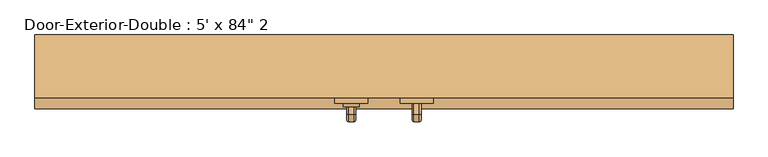
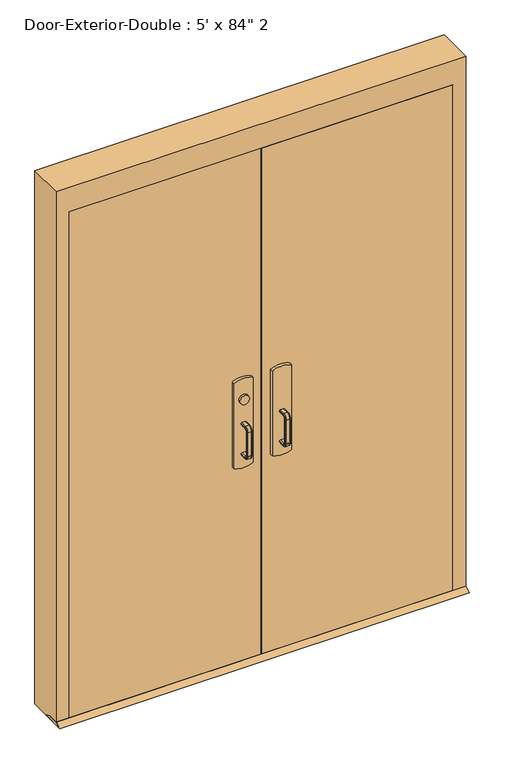
"""IFC4 building model written with IfcOpenShell, lengths in millimetres: door geometry."""

from ifc_helpers import new_model, si_unit, point, frame, frame_2d, origin, place, context, project, spatial, polyline, circle_curve, ellipse_curve, trimmed, segment, composite_curve, outline, extrude, faceted_brep, source, transform, mapped, element, save
from ifc_brep_helpers import plane_surface, cylinder_surface, revolved_surface, advanced_brep


def door_253b1ced(model_context):
    return source(origin(), model_context, "Body", "SolidModel", [
        extrude(outline(polyline([(-474.1333333, 12.7), (-76.2, 12.7), (-76.2, 6.35), (-474.1333333, 6.35), (-474.1333333, 12.7)])), frame((0.0, 0.0, 990.6), z_axis=(0.0, 0.0, 1.0), x_axis=(1.0, 0.0, 0.0)), (0.0, 0.0, 1.0), 50.8),
        advanced_brep(
        [(-12.7, 6.35, 1041.4), (-12.7, 6.35, 990.6), (-76.2, 6.35, 990.6), (-673.1, 6.35, 990.6), (-673.1, 6.35, 1041.4), (-76.2, 6.35, 1041.4), (-673.1, -25.4, 1041.4), (-673.1, -25.4, 990.6), (-76.2, -25.4, 990.6), (-76.2, -25.4, 927.1), (-57.15, -25.4, 908.05), (-31.75, -25.4, 908.05), (-12.7, -25.4, 927.1), (-12.7, -25.4, 1104.9), (-31.75, -25.4, 1123.95), (-57.15, -25.4, 1123.95), (-76.2, -25.4, 1104.9), (-76.2, -25.4, 1041.4), (-76.2, 3.1747533, 1041.4), (-12.7, 3.1747533, 1041.4), (-12.7, -1.8354269, 1104.9), (-12.7, -1.8354269, 927.1), (-12.7, 3.1747533, 990.6), (-76.2, 3.1747533, 990.6), (-76.2, -1.8354269, 1104.9), (-76.2, -1.8354269, 927.1), (-31.75, -3.338481, 1123.95), (-57.15, -3.338481, 1123.95), (-57.15, -3.338481, 908.05), (-31.75, -3.338481, 908.05)],
        [
            (0, 1),
            (1, 2),
            (2, 3),
            (3, 4),
            (4, 5),
            (5, 0),
            (6, 7),
            (7, 8),
            (8, 9),
            (9, 10, circle_curve(frame((-57.15, -25.4, 927.1), z_axis=(0.0, -1.0, 0.0), x_axis=(-1.0, 0.0, 0.0)), 19.05)),
            (10, 11),
            (11, 12, circle_curve(frame((-31.75, -25.4, 927.1), z_axis=(0.0, -1.0, 0.0), x_axis=(-1.0, 0.0, 0.0)), 19.05)),
            (12, 13),
            (13, 14, circle_curve(frame((-31.75, -25.4, 1104.9), z_axis=(0.0, -1.0, 0.0), x_axis=(-1.0, 0.0, 0.0)), 19.05)),
            (14, 15),
            (15, 16, circle_curve(frame((-57.15, -25.4, 1104.9), z_axis=(0.0, -1.0, 0.0), x_axis=(-1.0, 0.0, 0.0)), 19.05)),
            (16, 17),
            (17, 6),
            (4, 6),
            (17, 18),
            (18, 19),
            (19, 0),
            (19, 20),
            (20, 13),
            (12, 21),
            (21, 22),
            (22, 1),
            (7, 3),
            (22, 23),
            (23, 8),
            (16, 24),
            (24, 18),
            (23, 25),
            (25, 9),
            (14, 26),
            (26, 27),
            (27, 15),
            (10, 28),
            (28, 29),
            (29, 11),
            (25, 28, ellipse_curve(frame((-57.15, -1.8354269, 927.1), z_axis=(0.0, -0.9969018152893365, 0.07865602756830282), x_axis=(0.0, 0.07865602756830208, 0.9969018152893365)), 19.1092038, 19.05)),
            (27, 24, ellipse_curve(frame((-57.15, -1.8354269, 1104.9), z_axis=(0.0, -0.9969018152893376, -0.07865602756828934), x_axis=(0.0, 0.078656027568288, -0.9969018152893377)), 19.1092038, 19.05)),
            (20, 26, ellipse_curve(frame((-31.75, -1.8354269, 1104.9), z_axis=(0.0, -0.9969018152893376, -0.07865602756828934), x_axis=(0.0, 0.078656027568288, -0.9969018152893377)), 19.1092038, 19.05)),
            (29, 21, ellipse_curve(frame((-31.75, -1.8354269, 927.1), z_axis=(0.0, -0.9969018152893365, 0.07865602756830282), x_axis=(0.0, 0.07865602756830208, 0.9969018152893365)), 19.1092038, 19.05)),
        ],
        [
            plane_surface(frame((-12.7, 6.35, 1041.4), z_axis=(0.0, 1.0, 0.0), x_axis=(1.0, 0.0, 0.0))),
            plane_surface(frame((-12.7, -25.4, 1041.4), z_axis=(0.0, -1.0, 0.0), x_axis=(-1.0, 0.0, 0.0))),
            plane_surface(frame((-673.1, 6.35, 1041.4), z_axis=(0.0, 0.0, 1.0), x_axis=(0.0, -1.0, 0.0))),
            plane_surface(frame((-12.7, 6.35, 1041.4), z_axis=(1.0, 0.0, 0.0), x_axis=(0.0, -1.0, 0.0))),
            plane_surface(frame((-12.7, 6.35, 990.6), z_axis=(0.0, 0.0, -1.0), x_axis=(0.0, -1.0, 0.0))),
            plane_surface(frame((-673.1, 6.35, 990.6), z_axis=(-1.0, 0.0, 0.0), x_axis=(0.0, -1.0, 0.0))),
            plane_surface(frame((-76.2, 3.1747533, 927.1), z_axis=(-1.0, 0.0, 0.0), x_axis=(0.0, -1.0, 0.0))),
            plane_surface(frame((-57.15, 3.1747533, 1123.95), z_axis=(0.0, 0.0, 1.0), x_axis=(0.0, -1.0, 0.0))),
            plane_surface(frame((-31.75, 3.1747533, 908.05), z_axis=(0.0, 0.0, -1.0), x_axis=(0.0, -1.0, 0.0))),
            cylinder_surface(frame((-57.15, -25.4, 927.1), z_axis=(0.0, 1.0, 0.0), x_axis=(-1.0, 0.0, 0.0)), 19.05),
            cylinder_surface(frame((-57.15, -25.4, 1104.9), z_axis=(0.0, 1.0, 0.0), x_axis=(-1.0, 0.0, 0.0)), 19.05),
            cylinder_surface(frame((-31.75, -25.4, 1104.9), z_axis=(0.0, 1.0, 0.0), x_axis=(-1.0, 0.0, 0.0)), 19.05),
            cylinder_surface(frame((-31.75, -25.4, 927.1), z_axis=(0.0, 1.0, 0.0), x_axis=(-1.0, 0.0, 0.0)), 19.05),
            plane_surface(frame((-76.2, 3.1747533, 1041.4), z_axis=(0.0, 0.9969018152893376, 0.07865602756828934), x_axis=(1.0, 0.0, 0.0))),
            plane_surface(frame((-76.2, -3.338481, 908.05), z_axis=(0.0, 0.9969018152893365, -0.07865602756830282), x_axis=(1.0, 0.0, 0.0))),
        ],
        [
            (0, [[1, 2, 3, 4, 5, 6]]),
            (1, [[7, 8, 9, 10, 11, 12, 13, 14, 15, 16, 17, 18]]),
            (2, [[19, -18, 20, 21, 22, -6, -5]]),
            (3, [[-1, -22, 23, 24, -13, 25, 26, 27]]),
            (4, [[28, -3, -2, -27, 29, 30, -8]]),
            (5, [[-4, -28, -7, -19]]),
            (6, [[-17, 31, 32, -20]]),
            (6, [[-9, -30, 33, 34]]),
            (7, [[-15, 35, 36, 37]]),
            (8, [[-11, 38, 39, 40]]),
            (9, [[-10, -34, 41, -38]]),
            (10, [[-16, -37, 42, -31]]),
            (11, [[-14, -24, 43, -35]]),
            (12, [[-12, -40, 44, -25]]),
            (13, [[-21, -32, -42, -36, -43, -23]]),
            (14, [[-26, -44, -39, -41, -33, -29]]),
        ],
    ),
        extrude(outline(polyline([(-69.85, 12.7), (-25.4, 12.7), (0.0, 0.0), (-95.25, 0.0), (-69.85, 12.7)])), frame((-812.8, 0.0, 0.0), z_axis=(1.0, 0.0, 0.0), x_axis=(0.0, 1.0, 0.0)), (0.0, 0.0, 1.0), 1625.6),
        extrude(outline(polyline([(474.1333333, 12.7), (474.1333333, 6.35), (76.2, 6.35), (76.2, 12.7), (474.1333333, 12.7)])), frame((0.0, 0.0, 990.6), z_axis=(0.0, 0.0, 1.0), x_axis=(1.0, 0.0, 0.0)), (0.0, 0.0, 1.0), 50.8),
        advanced_brep(
        [(12.7, 6.35, 1041.4), (76.2, 6.35, 1041.4), (673.1, 6.35, 1041.4), (673.1, 6.35, 990.6), (76.2, 6.35, 990.6), (12.7, 6.35, 990.6), (673.1, -25.4, 1041.4), (76.2, -25.4, 1041.4), (76.2, -25.4, 1104.9), (57.15, -25.4, 1123.95), (31.75, -25.4, 1123.95), (12.7, -25.4, 1104.9), (12.7, -25.4, 927.1), (31.75, -25.4, 908.05), (57.15, -25.4, 908.05), (76.2, -25.4, 927.1), (76.2, -25.4, 990.6), (673.1, -25.4, 990.6), (12.7, 3.1747533, 1041.4), (76.2, 3.1747533, 1041.4), (12.7, 3.1747533, 990.6), (12.7, -1.8354269, 927.1), (12.7, -1.8354269, 1104.9), (76.2, 3.1747533, 990.6), (76.2, -1.8354269, 1104.9), (76.2, -1.8354269, 927.1), (57.15, -3.338481, 1123.95), (31.75, -3.338481, 1123.95), (31.75, -3.338481, 908.05), (57.15, -3.338481, 908.05)],
        [
            (0, 1),
            (1, 2),
            (2, 3),
            (3, 4),
            (4, 5),
            (5, 0),
            (6, 7),
            (7, 8),
            (8, 9, circle_curve(frame((57.15, -25.4, 1104.9), z_axis=(0.0, -1.0, 0.0), x_axis=(1.0, 0.0, 0.0)), 19.05)),
            (9, 10),
            (10, 11, circle_curve(frame((31.75, -25.4, 1104.9), z_axis=(0.0, -1.0, 0.0), x_axis=(1.0, 0.0, 0.0)), 19.05)),
            (11, 12),
            (12, 13, circle_curve(frame((31.75, -25.4, 927.1), z_axis=(0.0, -1.0, 0.0), x_axis=(1.0, 0.0, 0.0)), 19.05)),
            (13, 14),
            (14, 15, circle_curve(frame((57.15, -25.4, 927.1), z_axis=(0.0, -1.0, 0.0), x_axis=(1.0, 0.0, 0.0)), 19.05)),
            (15, 16),
            (16, 17),
            (17, 6),
            (0, 18),
            (18, 19),
            (19, 7),
            (6, 2),
            (5, 20),
            (20, 21),
            (21, 12),
            (11, 22),
            (22, 18),
            (16, 23),
            (23, 20),
            (3, 17),
            (19, 24),
            (24, 8),
            (15, 25),
            (25, 23),
            (9, 26),
            (26, 27),
            (27, 10),
            (13, 28),
            (28, 29),
            (29, 14),
            (29, 25, ellipse_curve(frame((57.15, -1.8354269, 927.1), z_axis=(0.0, -0.9969018152893365, 0.07865602756830282), x_axis=(0.0, 0.07865602756830208, 0.9969018152893365)), 19.1092038, 19.05)),
            (24, 26, ellipse_curve(frame((57.15, -1.8354269, 1104.9), z_axis=(0.0, -0.9969018152893376, -0.07865602756828934), x_axis=(0.0, 0.078656027568288, -0.9969018152893377)), 19.1092038, 19.05)),
            (27, 22, ellipse_curve(frame((31.75, -1.8354269, 1104.9), z_axis=(0.0, -0.9969018152893376, -0.07865602756828934), x_axis=(0.0, 0.078656027568288, -0.9969018152893377)), 19.1092038, 19.05)),
            (21, 28, ellipse_curve(frame((31.75, -1.8354269, 927.1), z_axis=(0.0, -0.9969018152893365, 0.07865602756830282), x_axis=(0.0, 0.07865602756830208, 0.9969018152893365)), 19.1092038, 19.05)),
        ],
        [
            plane_surface(frame((12.7, 6.35, 1041.4), z_axis=(0.0, 1.0, 0.0), x_axis=(-1.0, 0.0, 0.0))),
            plane_surface(frame((12.7, -25.4, 1041.4), z_axis=(0.0, -1.0, 0.0), x_axis=(1.0, 0.0, 0.0))),
            plane_surface(frame((673.1, 6.35, 1041.4), z_axis=(0.0, 0.0, 1.0), x_axis=(0.0, -1.0, 0.0))),
            plane_surface(frame((12.7, 6.35, 1041.4), z_axis=(-1.0, 0.0, 0.0), x_axis=(0.0, -1.0, 0.0))),
            plane_surface(frame((12.7, 6.35, 990.6), z_axis=(0.0, 0.0, -1.0), x_axis=(0.0, -1.0, 0.0))),
            plane_surface(frame((673.1, 6.35, 990.6), z_axis=(1.0, 0.0, 0.0), x_axis=(0.0, -1.0, 0.0))),
            plane_surface(frame((76.2, 3.1747533, 927.1), z_axis=(1.0, 0.0, 0.0), x_axis=(0.0, -1.0, 0.0))),
            plane_surface(frame((57.15, 3.1747533, 1123.95), z_axis=(0.0, 0.0, 1.0), x_axis=(0.0, -1.0, 0.0))),
            plane_surface(frame((31.75, 3.1747533, 908.05), z_axis=(0.0, 0.0, -1.0), x_axis=(0.0, -1.0, 0.0))),
            cylinder_surface(frame((57.15, -25.4, 927.1), z_axis=(0.0, 1.0, 0.0), x_axis=(1.0, 0.0, 0.0)), 19.05),
            cylinder_surface(frame((57.15, -25.4, 1104.9), z_axis=(0.0, 1.0, 0.0), x_axis=(1.0, 0.0, 0.0)), 19.05),
            cylinder_surface(frame((31.75, -25.4, 1104.9), z_axis=(0.0, 1.0, 0.0), x_axis=(1.0, 0.0, 0.0)), 19.05),
            cylinder_surface(frame((31.75, -25.4, 927.1), z_axis=(0.0, 1.0, 0.0), x_axis=(1.0, 0.0, 0.0)), 19.05),
            plane_surface(frame((76.2, 3.1747533, 1041.4), z_axis=(0.0, 0.9969018152893376, 0.07865602756828934), x_axis=(-1.0, 0.0, 0.0))),
            plane_surface(frame((76.2, -3.338481, 908.05), z_axis=(0.0, 0.9969018152893365, -0.07865602756830282), x_axis=(-1.0, 0.0, 0.0))),
        ],
        [
            (0, [[1, 2, 3, 4, 5, 6]]),
            (1, [[7, 8, 9, 10, 11, 12, 13, 14, 15, 16, 17, 18]]),
            (2, [[-2, -1, 19, 20, 21, -7, 22]]),
            (3, [[23, 24, 25, -12, 26, 27, -19, -6]]),
            (4, [[-17, 28, 29, -23, -5, -4, 30]]),
            (5, [[-22, -18, -30, -3]]),
            (6, [[-21, 31, 32, -8]]),
            (6, [[33, 34, -28, -16]]),
            (7, [[35, 36, 37, -10]]),
            (8, [[38, 39, 40, -14]]),
            (9, [[-40, 41, -33, -15]]),
            (10, [[-32, 42, -35, -9]]),
            (11, [[-37, 43, -26, -11]]),
            (12, [[-25, 44, -38, -13]]),
            (13, [[-27, -43, -36, -42, -31, -20]]),
            (14, [[-29, -34, -41, -39, -44, -24]]),
        ],
    ),
        advanced_brep(
        [(66.2, -82.55, 1017.190625), (69.771875, -82.55, 1020.7625), (82.628125, -82.55, 1020.7625), (86.2, -82.55, 1017.190625), (86.2, -82.55, 1014.8090406), (82.6284594, -82.55, 1011.2375), (69.771875, -82.55, 1011.2375), (66.2, -82.55, 1014.809375), (66.2, -82.55, 887.809375), (66.2, -82.55, 890.190625), (69.771875, -82.55, 893.7625), (82.6284594, -82.55, 893.7625), (86.2, -82.55, 890.1909594), (86.2, -82.55, 887.809375), (82.628125, -82.55, 884.2375), (69.771875, -82.55, 884.2375), (66.2, -107.95, 1014.809375), (66.2, -119.459375, 1003.3), (66.2, -119.459375, 901.7), (66.2, -107.95, 890.190625), (66.2, -107.95, 887.809375), (66.2, -121.840625, 901.7), (66.2, -121.840625, 1003.3), (66.2, -107.95, 1017.190625), (69.771875, -107.95, 1011.2375), (82.6284594, -107.95, 1011.2375), (86.2, -107.95, 1014.8090406), (86.2, -107.95, 1017.190625), (86.2, -121.840625, 1003.3), (86.2, -121.840625, 901.7), (86.2, -107.95, 887.809375), (86.2, -107.95, 890.1909594), (86.2, -119.4590406, 901.7), (86.2, -119.4590406, 1003.3), (82.628125, -107.95, 1020.7625), (69.771875, -107.95, 1020.7625), (69.771875, -115.8875, 1003.3), (82.6284594, -115.8875, 1003.3), (82.628125, -125.4125, 1003.3), (69.771875, -125.4125, 1003.3), (69.771875, -115.8875, 901.7), (82.6284594, -115.8875, 901.7), (82.628125, -125.4125, 901.7), (69.771875, -125.4125, 901.7), (69.771875, -107.95, 893.7625), (82.6284594, -107.95, 893.7625), (82.628125, -107.95, 884.2375), (69.771875, -107.95, 884.2375)],
        [
            (0, 1, circle_curve(frame((69.771875, -82.55, 1017.190625), z_axis=(0.0, 1.0, 0.0), x_axis=(0.0, 0.0, 1.0)), 3.571875)),
            (1, 2),
            (2, 3, circle_curve(frame((82.628125, -82.55, 1017.190625), z_axis=(0.0, 1.0, 0.0), x_axis=(0.0, 0.0, 1.0)), 3.571875)),
            (3, 4),
            (4, 5, circle_curve(frame((82.6284594, -82.55, 1014.8090406), z_axis=(0.0, 1.0, 0.0), x_axis=(0.0, 0.0, 1.0)), 3.5715406)),
            (5, 6),
            (6, 7, circle_curve(frame((69.771875, -82.55, 1014.809375), z_axis=(0.0, 1.0, 0.0), x_axis=(0.0, 0.0, 1.0)), 3.571875)),
            (7, 0),
            (8, 9),
            (9, 10, circle_curve(frame((69.771875, -82.55, 890.190625), z_axis=(0.0, 1.0, 0.0), x_axis=(0.0, 0.0, -1.0)), 3.571875)),
            (10, 11),
            (11, 12, circle_curve(frame((82.6284594, -82.55, 890.1909594), z_axis=(0.0, 1.0, 0.0), x_axis=(0.0, 0.0, -1.0)), 3.5715406)),
            (12, 13),
            (13, 14, circle_curve(frame((82.628125, -82.55, 887.809375), z_axis=(0.0, 1.0, 0.0), x_axis=(0.0, 0.0, -1.0)), 3.571875)),
            (14, 15),
            (15, 8, circle_curve(frame((69.771875, -82.55, 887.809375), z_axis=(0.0, 1.0, 0.0), x_axis=(0.0, 0.0, -1.0)), 3.571875)),
            (7, 16),
            (16, 17, circle_curve(frame((66.2, -107.95, 1003.3), z_axis=(1.0, 0.0, 0.0), x_axis=(0.0, 0.0, 1.0)), 11.509375)),
            (17, 18),
            (18, 19, circle_curve(frame((66.2, -107.95, 901.7), z_axis=(1.0, 0.0, 0.0), x_axis=(0.0, -1.0, 0.0)), 11.509375)),
            (19, 9),
            (8, 20),
            (20, 21, circle_curve(frame((66.2, -107.95, 901.7), z_axis=(-1.0, 0.0, 0.0), x_axis=(0.0, -1.0, 0.0)), 13.890625)),
            (21, 22),
            (22, 23, circle_curve(frame((66.2, -107.95, 1003.3), z_axis=(-1.0, 0.0, 0.0), x_axis=(0.0, 0.0, 1.0)), 13.890625)),
            (23, 0),
            (6, 24),
            (24, 16, circle_curve(frame((69.771875, -107.95, 1014.809375), z_axis=(0.0, 1.0, 0.0), x_axis=(0.0, 0.0, 1.0)), 3.571875)),
            (5, 25),
            (25, 24),
            (4, 26),
            (26, 25, circle_curve(frame((82.6284594, -107.95, 1014.8090406), z_axis=(0.0, 1.0, 0.0), x_axis=(0.0, 0.0, 1.0)), 3.5715406)),
            (3, 27),
            (27, 28, circle_curve(frame((86.2, -107.95, 1003.3), z_axis=(1.0, 0.0, 0.0), x_axis=(0.0, 0.0, 1.0)), 13.890625)),
            (28, 29),
            (29, 30, circle_curve(frame((86.2, -107.95, 901.7), z_axis=(1.0, 0.0, 0.0), x_axis=(0.0, -1.0, 0.0)), 13.890625)),
            (30, 13),
            (12, 31),
            (31, 32, circle_curve(frame((86.2, -107.95, 901.7), z_axis=(-1.0, 0.0, 0.0), x_axis=(0.0, -1.0, 0.0)), 11.5090406)),
            (32, 33),
            (33, 26, circle_curve(frame((86.2, -107.95, 1003.3), z_axis=(-1.0, 0.0, 0.0), x_axis=(0.0, 0.0, 1.0)), 11.5090406)),
            (2, 34),
            (34, 27, circle_curve(frame((82.628125, -107.95, 1017.190625), z_axis=(0.0, 1.0, 0.0), x_axis=(0.0, 0.0, 1.0)), 3.571875)),
            (1, 35),
            (35, 34),
            (23, 35, circle_curve(frame((69.771875, -107.95, 1017.190625), z_axis=(0.0, 1.0, 0.0), x_axis=(0.0, 0.0, 1.0)), 3.571875)),
            (36, 17, circle_curve(frame((69.771875, -119.459375, 1003.3), z_axis=(0.0, 0.0, 1.0), x_axis=(0.0, -1.0, 0.0)), 3.571875)),
            (24, 36, circle_curve(frame((69.771875, -107.95, 1003.3), z_axis=(1.0, 0.0, 0.0), x_axis=(0.0, 0.0, 1.0)), 7.9375)),
            (37, 36),
            (25, 37, circle_curve(frame((82.6284594, -107.95, 1003.3), z_axis=(1.0, 0.0, 0.0), x_axis=(0.0, 0.0, 1.0)), 7.9375)),
            (33, 37, circle_curve(frame((82.6284594, -119.4590406, 1003.3), z_axis=(0.0, 0.0, 1.0), x_axis=(0.0, -1.0, 0.0)), 3.5715406)),
            (38, 28, circle_curve(frame((82.628125, -121.840625, 1003.3), z_axis=(0.0, 0.0, 1.0), x_axis=(0.0, -1.0, 0.0)), 3.571875)),
            (34, 38, circle_curve(frame((82.628125, -107.95, 1003.3), z_axis=(1.0, 0.0, 0.0), x_axis=(0.0, 0.0, 1.0)), 17.4625)),
            (39, 38),
            (35, 39, circle_curve(frame((69.771875, -107.95, 1003.3), z_axis=(1.0, 0.0, 0.0), x_axis=(0.0, 0.0, 1.0)), 17.4625)),
            (22, 39, circle_curve(frame((69.771875, -121.840625, 1003.3), z_axis=(0.0, 0.0, 1.0), x_axis=(0.0, -1.0, 0.0)), 3.571875)),
            (36, 40),
            (40, 18, circle_curve(frame((69.771875, -119.459375, 901.7), z_axis=(0.0, 0.0, 1.0), x_axis=(0.0, -1.0, 0.0)), 3.571875)),
            (37, 41),
            (41, 40),
            (32, 41, circle_curve(frame((82.6284594, -119.4590406, 901.7), z_axis=(0.0, 0.0, 1.0), x_axis=(0.0, -1.0, 0.0)), 3.5715406)),
            (38, 42),
            (42, 29, circle_curve(frame((82.628125, -121.840625, 901.7), z_axis=(0.0, 0.0, 1.0), x_axis=(0.0, -1.0, 0.0)), 3.571875)),
            (39, 43),
            (43, 42),
            (21, 43, circle_curve(frame((69.771875, -121.840625, 901.7), z_axis=(0.0, 0.0, 1.0), x_axis=(0.0, -1.0, 0.0)), 3.571875)),
            (44, 19, circle_curve(frame((69.771875, -107.95, 890.190625), z_axis=(0.0, -1.0, 0.0), x_axis=(0.0, 0.0, -1.0)), 3.571875)),
            (40, 44, circle_curve(frame((69.771875, -107.95, 901.7), z_axis=(1.0, 0.0, 0.0), x_axis=(0.0, -1.0, 0.0)), 7.9375)),
            (45, 44),
            (41, 45, circle_curve(frame((82.6284594, -107.95, 901.7), z_axis=(1.0, 0.0, 0.0), x_axis=(0.0, -1.0, 0.0)), 7.9375)),
            (31, 45, circle_curve(frame((82.6284594, -107.95, 890.1909594), z_axis=(0.0, -1.0, 0.0), x_axis=(0.0, 0.0, -1.0)), 3.5715406)),
            (46, 30, circle_curve(frame((82.628125, -107.95, 887.809375), z_axis=(0.0, -1.0, 0.0), x_axis=(0.0, 0.0, -1.0)), 3.571875)),
            (42, 46, circle_curve(frame((82.628125, -107.95, 901.7), z_axis=(1.0, 0.0, 0.0), x_axis=(0.0, -1.0, 0.0)), 17.4625)),
            (47, 46),
            (43, 47, circle_curve(frame((69.771875, -107.95, 901.7), z_axis=(1.0, 0.0, 0.0), x_axis=(0.0, -1.0, 0.0)), 17.4625)),
            (20, 47, circle_curve(frame((69.771875, -107.95, 887.809375), z_axis=(0.0, -1.0, 0.0), x_axis=(0.0, 0.0, -1.0)), 3.571875)),
            (44, 10),
            (45, 11),
            (46, 14),
            (47, 15),
        ],
        [
            plane_surface(frame((76.2, -82.55, 1016.0), z_axis=(0.0, 1.0, 0.0), x_axis=(1.0, 0.0, 0.0))),
            plane_surface(frame((76.2, -82.55, 889.0), z_axis=(0.0, 1.0, 0.0), x_axis=(1.0, 0.0, 0.0))),
            plane_surface(frame((66.2, -82.55, 1017.190625), z_axis=(-1.0, 0.0, 0.0), x_axis=(0.0, -1.0, 0.0))),
            cylinder_surface(frame((69.771875, -82.55, 1014.809375), z_axis=(0.0, 1.0, 0.0), x_axis=(0.0, 0.0, 1.0)), 3.571875),
            plane_surface(frame((69.771875, -82.55, 1011.2375), z_axis=(0.0, 0.0, -1.0), x_axis=(0.0, -1.0, 0.0))),
            cylinder_surface(frame((82.6284594, -82.55, 1014.8090406), z_axis=(0.0, 1.0, 0.0), x_axis=(0.0, 0.0, 1.0)), 3.5715406),
            plane_surface(frame((86.2, -82.55, 1014.8090406), z_axis=(1.0, 0.0, 0.0), x_axis=(0.0, -1.0, 0.0))),
            cylinder_surface(frame((82.628125, -82.55, 1017.190625), z_axis=(0.0, 1.0, 0.0), x_axis=(0.0, 0.0, 1.0)), 3.571875),
            plane_surface(frame((82.628125, -82.55, 1020.7625), z_axis=(0.0, 0.0, 1.0), x_axis=(0.0, -1.0, 0.0))),
            cylinder_surface(frame((69.771875, -82.55, 1017.190625), z_axis=(0.0, 1.0, 0.0), x_axis=(0.0, 0.0, 1.0)), 3.571875),
            revolved_surface(trimmed(ellipse_curve(frame((69.771875, -107.95, 1014.809375), z_axis=(0.0, -1.0, 0.0), x_axis=(0.0, 0.0, 1.0)), 3.571875, 3.571875), [point((66.2, -107.95, 1014.809375))], [point((69.771875, -107.95, 1011.2375))], True, "CARTESIAN"), (76.2, -107.95, 1003.3), (-1.0, 0.0, 0.0)),
            revolved_surface(polyline([(69.771875, -107.95, 1011.2375), (82.6284594, -107.95, 1011.2375)]), (76.2, -107.95, 1003.3), (-1.0, 0.0, 0.0)),
            revolved_surface(trimmed(ellipse_curve(frame((82.6284594, -107.95, 1014.8090406), z_axis=(0.0, -1.0, 0.0), x_axis=(0.0, 0.0, 1.0)), 3.5715406, 3.5715406), [point((82.6284594, -107.95, 1011.2375))], [point((86.2, -107.95, 1014.8090406))], True, "CARTESIAN"), (76.2, -107.95, 1003.3), (-1.0, 0.0, 0.0)),
            revolved_surface(trimmed(ellipse_curve(frame((82.628125, -107.95, 1017.190625), z_axis=(0.0, -1.0, 0.0), x_axis=(0.0, 0.0, 1.0)), 3.571875, 3.571875), [point((86.2, -107.95, 1017.190625))], [point((82.628125, -107.95, 1020.7625))], True, "CARTESIAN"), (76.2, -107.95, 1003.3), (-1.0, 0.0, 0.0)),
            cylinder_surface(frame((76.2, -107.95, 1003.3), z_axis=(-1.0, 0.0, 0.0), x_axis=(0.0, 0.0, 1.0)), 17.4625),
            revolved_surface(trimmed(ellipse_curve(frame((69.771875, -107.95, 1017.190625), z_axis=(0.0, -1.0, 0.0), x_axis=(0.0, 0.0, 1.0)), 3.571875, 3.571875), [point((69.771875, -107.95, 1020.7625))], [point((66.2, -107.95, 1017.190625))], True, "CARTESIAN"), (76.2, -107.95, 1003.3), (-1.0, 0.0, 0.0)),
            cylinder_surface(frame((69.771875, -119.459375, 1003.3), z_axis=(0.0, 0.0, 1.0), x_axis=(0.0, -1.0, 0.0)), 3.571875),
            plane_surface(frame((69.771875, -115.8875, 1003.3), z_axis=(0.0, 1.0, 0.0), x_axis=(0.0, 0.0, -1.0))),
            cylinder_surface(frame((82.6284594, -119.4590406, 1003.3), z_axis=(0.0, 0.0, 1.0), x_axis=(0.0, -1.0, 0.0)), 3.5715406),
            cylinder_surface(frame((82.628125, -121.840625, 1003.3), z_axis=(0.0, 0.0, 1.0), x_axis=(0.0, -1.0, 0.0)), 3.571875),
            plane_surface(frame((82.628125, -125.4125, 1003.3), z_axis=(0.0, -1.0, 0.0), x_axis=(0.0, 0.0, -1.0))),
            cylinder_surface(frame((69.771875, -121.840625, 1003.3), z_axis=(0.0, 0.0, 1.0), x_axis=(0.0, -1.0, 0.0)), 3.571875),
            revolved_surface(trimmed(ellipse_curve(frame((69.771875, -119.459375, 901.7), z_axis=(0.0, 0.0, -1.0), x_axis=(0.0, -1.0, 0.0)), 3.571875, 3.571875), [point((66.2, -119.459375, 901.7))], [point((69.771875, -115.8875, 901.7))], True, "CARTESIAN"), (76.2, -107.95, 901.7), (-1.0, 0.0, 0.0)),
            revolved_surface(polyline([(69.771875, -115.8875, 901.7), (82.6284594, -115.8875, 901.7)]), (76.2, -107.95, 901.7), (-1.0, 0.0, 0.0)),
            revolved_surface(trimmed(ellipse_curve(frame((82.6284594, -119.4590406, 901.7), z_axis=(0.0, 0.0, -1.0), x_axis=(0.0, -1.0, 0.0)), 3.5715406, 3.5715406), [point((82.6284594, -115.8875, 901.7))], [point((86.2, -119.4590406, 901.7))], True, "CARTESIAN"), (76.2, -107.95, 901.7), (-1.0, 0.0, 0.0)),
            revolved_surface(trimmed(ellipse_curve(frame((82.628125, -121.840625, 901.7), z_axis=(0.0, 0.0, -1.0), x_axis=(0.0, -1.0, 0.0)), 3.571875, 3.571875), [point((86.2, -121.840625, 901.7))], [point((82.628125, -125.4125, 901.7))], True, "CARTESIAN"), (76.2, -107.95, 901.7), (-1.0, 0.0, 0.0)),
            cylinder_surface(frame((76.2, -107.95, 901.7), z_axis=(-1.0, 0.0, 0.0), x_axis=(0.0, -1.0, 0.0)), 17.4625),
            revolved_surface(trimmed(ellipse_curve(frame((69.771875, -121.840625, 901.7), z_axis=(0.0, 0.0, -1.0), x_axis=(0.0, -1.0, 0.0)), 3.571875, 3.571875), [point((69.771875, -125.4125, 901.7))], [point((66.2, -121.840625, 901.7))], True, "CARTESIAN"), (76.2, -107.95, 901.7), (-1.0, 0.0, 0.0)),
            cylinder_surface(frame((69.771875, -107.95, 890.190625), z_axis=(0.0, -1.0, 0.0), x_axis=(0.0, 0.0, -1.0)), 3.571875),
            plane_surface(frame((69.771875, -107.95, 893.7625), z_axis=(0.0, 0.0, 1.0), x_axis=(0.0, 1.0, 0.0))),
            cylinder_surface(frame((82.6284594, -107.95, 890.1909594), z_axis=(0.0, -1.0, 0.0), x_axis=(0.0, 0.0, -1.0)), 3.5715406),
            cylinder_surface(frame((82.628125, -107.95, 887.809375), z_axis=(0.0, -1.0, 0.0), x_axis=(0.0, 0.0, -1.0)), 3.571875),
            plane_surface(frame((82.628125, -107.95, 884.2375), z_axis=(0.0, 0.0, -1.0), x_axis=(0.0, 1.0, 0.0))),
            cylinder_surface(frame((69.771875, -107.95, 887.809375), z_axis=(0.0, -1.0, 0.0), x_axis=(0.0, 0.0, -1.0)), 3.571875),
        ],
        [
            (0, [[1, 2, 3, 4, 5, 6, 7, 8]]),
            (1, [[9, 10, 11, 12, 13, 14, 15, 16]]),
            (2, [[17, 18, 19, 20, 21, -9, 22, 23, 24, 25, 26, -8]]),
            (3, [[27, 28, -17, -7]]),
            (4, [[29, 30, -27, -6]]),
            (5, [[31, 32, -29, -5]]),
            (6, [[33, 34, 35, 36, 37, -13, 38, 39, 40, 41, -31, -4]]),
            (7, [[42, 43, -33, -3]]),
            (8, [[44, 45, -42, -2]]),
            (9, [[-26, 46, -44, -1]]),
            (10, [[47, -18, -28, 48]]),
            (11, [[49, -48, -30, 50]]),
            (12, [[51, -50, -32, -41]]),
            (13, [[52, -34, -43, 53]]),
            (14, [[54, -53, -45, 55]]),
            (15, [[56, -55, -46, -25]]),
            (16, [[57, 58, -19, -47]]),
            (17, [[59, 60, -57, -49]]),
            (18, [[-40, 61, -59, -51]]),
            (19, [[62, 63, -35, -52]]),
            (20, [[64, 65, -62, -54]]),
            (21, [[-24, 66, -64, -56]]),
            (22, [[67, -20, -58, 68]]),
            (23, [[69, -68, -60, 70]]),
            (24, [[71, -70, -61, -39]]),
            (25, [[72, -36, -63, 73]]),
            (26, [[74, -73, -65, 75]]),
            (27, [[76, -75, -66, -23]]),
            (28, [[77, -10, -21, -67]]),
            (29, [[78, -11, -77, -69]]),
            (30, [[-38, -12, -78, -71]]),
            (31, [[79, -14, -37, -72]]),
            (32, [[80, -15, -79, -74]]),
            (33, [[-22, -16, -80, -76]]),
        ],
    ),
        extrude(outline(composite_curve([segment(trimmed(circle_curve(frame_2d((1113.0338574, 76.2)), 89.3016225), [point((1193.8, 114.3))], [point((1193.8, 38.1))], False, "CARTESIAN"), True, "CONTINUOUS"), segment(polyline([(1193.8, 38.1), (838.2, 38.1)]), True, "CONTINUOUS"), segment(trimmed(circle_curve(frame_2d((918.9661426, 76.2)), 89.3016225), [point((838.2, 38.1))], [point((838.2, 114.3))], False, "CARTESIAN"), True, "CONTINUOUS"), segment(polyline([(838.2, 114.3), (1193.8, 114.3)]), True, "CONTINUOUS")], self_intersect=False)), frame((0.0, -82.55, 0.0), z_axis=(0.0, 1.0, 0.0), x_axis=(0.0, 0.0, 1.0)), (0.0, 0.0, 1.0), 12.7),
        advanced_brep(
        [(-86.2, -82.55, 1017.190625), (-82.628125, -82.55, 1020.7625), (-69.771875, -82.55, 1020.7625), (-66.2, -82.55, 1017.190625), (-66.2, -82.55, 1014.8090406), (-69.7715406, -82.55, 1011.2375), (-82.628125, -82.55, 1011.2375), (-86.2, -82.55, 1014.809375), (-86.2, -82.55, 887.809375), (-86.2, -82.55, 890.190625), (-82.628125, -82.55, 893.7625), (-69.7715406, -82.55, 893.7625), (-66.2, -82.55, 890.1909594), (-66.2, -82.55, 887.809375), (-69.771875, -82.55, 884.2375), (-82.628125, -82.55, 884.2375), (-86.2, -107.95, 1014.809375), (-86.2, -119.459375, 1003.3), (-86.2, -119.459375, 901.7), (-86.2, -107.95, 890.190625), (-86.2, -107.95, 887.809375), (-86.2, -121.840625, 901.7), (-86.2, -121.840625, 1003.3), (-86.2, -107.95, 1017.190625), (-82.628125, -107.95, 1011.2375), (-69.7715406, -107.95, 1011.2375), (-66.2, -107.95, 1014.8090406), (-66.2, -107.95, 1017.190625), (-66.2, -121.840625, 1003.3), (-66.2, -121.840625, 901.7), (-66.2, -107.95, 887.809375), (-66.2, -107.95, 890.1909594), (-66.2, -119.4590406, 901.7), (-66.2, -119.4590406, 1003.3), (-69.771875, -107.95, 1020.7625), (-82.628125, -107.95, 1020.7625), (-82.628125, -115.8875, 1003.3), (-69.7715406, -115.8875, 1003.3), (-69.771875, -125.4125, 1003.3), (-82.628125, -125.4125, 1003.3), (-82.628125, -115.8875, 901.7), (-69.7715406, -115.8875, 901.7), (-69.771875, -125.4125, 901.7), (-82.628125, -125.4125, 901.7), (-82.628125, -107.95, 893.7625), (-69.7715406, -107.95, 893.7625), (-69.771875, -107.95, 884.2375), (-82.628125, -107.95, 884.2375)],
        [
            (0, 1, circle_curve(frame((-82.628125, -82.55, 1017.190625), z_axis=(0.0, 1.0, 0.0), x_axis=(0.0, 0.0, 1.0)), 3.571875)),
            (1, 2),
            (2, 3, circle_curve(frame((-69.771875, -82.55, 1017.190625), z_axis=(0.0, 1.0, 0.0), x_axis=(0.0, 0.0, 1.0)), 3.571875)),
            (3, 4),
            (4, 5, circle_curve(frame((-69.7715406, -82.55, 1014.8090406), z_axis=(0.0, 1.0, 0.0), x_axis=(0.0, 0.0, 1.0)), 3.5715406)),
            (5, 6),
            (6, 7, circle_curve(frame((-82.628125, -82.55, 1014.809375), z_axis=(0.0, 1.0, 0.0), x_axis=(0.0, 0.0, 1.0)), 3.571875)),
            (7, 0),
            (8, 9),
            (9, 10, circle_curve(frame((-82.628125, -82.55, 890.190625), z_axis=(0.0, 1.0, 0.0), x_axis=(0.0, 0.0, -1.0)), 3.571875)),
            (10, 11),
            (11, 12, circle_curve(frame((-69.7715406, -82.55, 890.1909594), z_axis=(0.0, 1.0, 0.0), x_axis=(0.0, 0.0, -1.0)), 3.5715406)),
            (12, 13),
            (13, 14, circle_curve(frame((-69.771875, -82.55, 887.809375), z_axis=(0.0, 1.0, 0.0), x_axis=(0.0, 0.0, -1.0)), 3.571875)),
            (14, 15),
            (15, 8, circle_curve(frame((-82.628125, -82.55, 887.809375), z_axis=(0.0, 1.0, 0.0), x_axis=(0.0, 0.0, -1.0)), 3.571875)),
            (7, 16),
            (16, 17, circle_curve(frame((-86.2, -107.95, 1003.3), z_axis=(1.0, 0.0, 0.0), x_axis=(0.0, 0.0, 1.0)), 11.509375)),
            (17, 18),
            (18, 19, circle_curve(frame((-86.2, -107.95, 901.7), z_axis=(1.0, 0.0, 0.0), x_axis=(0.0, -1.0, 0.0)), 11.509375)),
            (19, 9),
            (8, 20),
            (20, 21, circle_curve(frame((-86.2, -107.95, 901.7), z_axis=(-1.0, 0.0, 0.0), x_axis=(0.0, -1.0, 0.0)), 13.890625)),
            (21, 22),
            (22, 23, circle_curve(frame((-86.2, -107.95, 1003.3), z_axis=(-1.0, 0.0, 0.0), x_axis=(0.0, 0.0, 1.0)), 13.890625)),
            (23, 0),
            (6, 24),
            (24, 16, circle_curve(frame((-82.628125, -107.95, 1014.809375), z_axis=(0.0, 1.0, 0.0), x_axis=(0.0, 0.0, 1.0)), 3.571875)),
            (5, 25),
            (25, 24),
            (4, 26),
            (26, 25, circle_curve(frame((-69.7715406, -107.95, 1014.8090406), z_axis=(0.0, 1.0, 0.0), x_axis=(0.0, 0.0, 1.0)), 3.5715406)),
            (3, 27),
            (27, 28, circle_curve(frame((-66.2, -107.95, 1003.3), z_axis=(1.0, 0.0, 0.0), x_axis=(0.0, 0.0, 1.0)), 13.890625)),
            (28, 29),
            (29, 30, circle_curve(frame((-66.2, -107.95, 901.7), z_axis=(1.0, 0.0, 0.0), x_axis=(0.0, -1.0, 0.0)), 13.890625)),
            (30, 13),
            (12, 31),
            (31, 32, circle_curve(frame((-66.2, -107.95, 901.7), z_axis=(-1.0, 0.0, 0.0), x_axis=(0.0, -1.0, 0.0)), 11.5090406)),
            (32, 33),
            (33, 26, circle_curve(frame((-66.2, -107.95, 1003.3), z_axis=(-1.0, 0.0, 0.0), x_axis=(0.0, 0.0, 1.0)), 11.5090406)),
            (2, 34),
            (34, 27, circle_curve(frame((-69.771875, -107.95, 1017.190625), z_axis=(0.0, 1.0, 0.0), x_axis=(0.0, 0.0, 1.0)), 3.571875)),
            (1, 35),
            (35, 34),
            (23, 35, circle_curve(frame((-82.628125, -107.95, 1017.190625), z_axis=(0.0, 1.0, 0.0), x_axis=(0.0, 0.0, 1.0)), 3.571875)),
            (36, 17, circle_curve(frame((-82.628125, -119.459375, 1003.3), z_axis=(0.0, 0.0, 1.0), x_axis=(0.0, -1.0, 0.0)), 3.571875)),
            (24, 36, circle_curve(frame((-82.628125, -107.95, 1003.3), z_axis=(1.0, 0.0, 0.0), x_axis=(0.0, 0.0, 1.0)), 7.9375)),
            (37, 36),
            (25, 37, circle_curve(frame((-69.7715406, -107.95, 1003.3), z_axis=(1.0, 0.0, 0.0), x_axis=(0.0, 0.0, 1.0)), 7.9375)),
            (33, 37, circle_curve(frame((-69.7715406, -119.4590406, 1003.3), z_axis=(0.0, 0.0, 1.0), x_axis=(0.0, -1.0, 0.0)), 3.5715406)),
            (38, 28, circle_curve(frame((-69.771875, -121.840625, 1003.3), z_axis=(0.0, 0.0, 1.0), x_axis=(0.0, -1.0, 0.0)), 3.571875)),
            (34, 38, circle_curve(frame((-69.771875, -107.95, 1003.3), z_axis=(1.0, 0.0, 0.0), x_axis=(0.0, 0.0, 1.0)), 17.4625)),
            (39, 38),
            (35, 39, circle_curve(frame((-82.628125, -107.95, 1003.3), z_axis=(1.0, 0.0, 0.0), x_axis=(0.0, 0.0, 1.0)), 17.4625)),
            (22, 39, circle_curve(frame((-82.628125, -121.840625, 1003.3), z_axis=(0.0, 0.0, 1.0), x_axis=(0.0, -1.0, 0.0)), 3.571875)),
            (36, 40),
            (40, 18, circle_curve(frame((-82.628125, -119.459375, 901.7), z_axis=(0.0, 0.0, 1.0), x_axis=(0.0, -1.0, 0.0)), 3.571875)),
            (37, 41),
            (41, 40),
            (32, 41, circle_curve(frame((-69.7715406, -119.4590406, 901.7), z_axis=(0.0, 0.0, 1.0), x_axis=(0.0, -1.0, 0.0)), 3.5715406)),
            (38, 42),
            (42, 29, circle_curve(frame((-69.771875, -121.840625, 901.7), z_axis=(0.0, 0.0, 1.0), x_axis=(0.0, -1.0, 0.0)), 3.571875)),
            (39, 43),
            (43, 42),
            (21, 43, circle_curve(frame((-82.628125, -121.840625, 901.7), z_axis=(0.0, 0.0, 1.0), x_axis=(0.0, -1.0, 0.0)), 3.571875)),
            (44, 19, circle_curve(frame((-82.628125, -107.95, 890.190625), z_axis=(0.0, -1.0, 0.0), x_axis=(0.0, 0.0, -1.0)), 3.571875)),
            (40, 44, circle_curve(frame((-82.628125, -107.95, 901.7), z_axis=(1.0, 0.0, 0.0), x_axis=(0.0, -1.0, 0.0)), 7.9375)),
            (45, 44),
            (41, 45, circle_curve(frame((-69.7715406, -107.95, 901.7), z_axis=(1.0, 0.0, 0.0), x_axis=(0.0, -1.0, 0.0)), 7.9375)),
            (31, 45, circle_curve(frame((-69.7715406, -107.95, 890.1909594), z_axis=(0.0, -1.0, 0.0), x_axis=(0.0, 0.0, -1.0)), 3.5715406)),
            (46, 30, circle_curve(frame((-69.771875, -107.95, 887.809375), z_axis=(0.0, -1.0, 0.0), x_axis=(0.0, 0.0, -1.0)), 3.571875)),
            (42, 46, circle_curve(frame((-69.771875, -107.95, 901.7), z_axis=(1.0, 0.0, 0.0), x_axis=(0.0, -1.0, 0.0)), 17.4625)),
            (47, 46),
            (43, 47, circle_curve(frame((-82.628125, -107.95, 901.7), z_axis=(1.0, 0.0, 0.0), x_axis=(0.0, -1.0, 0.0)), 17.4625)),
            (20, 47, circle_curve(frame((-82.628125, -107.95, 887.809375), z_axis=(0.0, -1.0, 0.0), x_axis=(0.0, 0.0, -1.0)), 3.571875)),
            (44, 10),
            (45, 11),
            (46, 14),
            (47, 15),
        ],
        [
            plane_surface(frame((-76.2, -82.55, 1016.0), z_axis=(0.0, 1.0, 0.0), x_axis=(1.0, 0.0, 0.0))),
            plane_surface(frame((-76.2, -82.55, 889.0), z_axis=(0.0, 1.0, 0.0), x_axis=(1.0, 0.0, 0.0))),
            plane_surface(frame((-86.2, -82.55, 1017.190625), z_axis=(-1.0, 0.0, 0.0), x_axis=(0.0, -1.0, 0.0))),
            cylinder_surface(frame((-82.628125, -82.55, 1014.809375), z_axis=(0.0, 1.0, 0.0), x_axis=(0.0, 0.0, 1.0)), 3.571875),
            plane_surface(frame((-82.628125, -82.55, 1011.2375), z_axis=(0.0, 0.0, -1.0), x_axis=(0.0, -1.0, 0.0))),
            cylinder_surface(frame((-69.7715406, -82.55, 1014.8090406), z_axis=(0.0, 1.0, 0.0), x_axis=(0.0, 0.0, 1.0)), 3.5715406),
            plane_surface(frame((-66.2, -82.55, 1014.8090406), z_axis=(1.0, 0.0, 0.0), x_axis=(0.0, -1.0, 0.0))),
            cylinder_surface(frame((-69.771875, -82.55, 1017.190625), z_axis=(0.0, 1.0, 0.0), x_axis=(0.0, 0.0, 1.0)), 3.571875),
            plane_surface(frame((-69.771875, -82.55, 1020.7625), z_axis=(0.0, 0.0, 1.0), x_axis=(0.0, -1.0, 0.0))),
            cylinder_surface(frame((-82.628125, -82.55, 1017.190625), z_axis=(0.0, 1.0, 0.0), x_axis=(0.0, 0.0, 1.0)), 3.571875),
            revolved_surface(trimmed(ellipse_curve(frame((-82.628125, -107.95, 1014.809375), z_axis=(0.0, -1.0, 0.0), x_axis=(0.0, 0.0, 1.0)), 3.571875, 3.571875), [point((-86.2, -107.95, 1014.809375))], [point((-82.628125, -107.95, 1011.2375))], True, "CARTESIAN"), (-76.2, -107.95, 1003.3), (-1.0, 0.0, 0.0)),
            revolved_surface(polyline([(-82.628125, -107.95, 1011.2375), (-69.7715406, -107.95, 1011.2375)]), (-76.2, -107.95, 1003.3), (-1.0, 0.0, 0.0)),
            revolved_surface(trimmed(ellipse_curve(frame((-69.7715406, -107.95, 1014.8090406), z_axis=(0.0, -1.0, 0.0), x_axis=(0.0, 0.0, 1.0)), 3.5715406, 3.5715406), [point((-69.7715406, -107.95, 1011.2375))], [point((-66.2, -107.95, 1014.8090406))], True, "CARTESIAN"), (-76.2, -107.95, 1003.3), (-1.0, 0.0, 0.0)),
            revolved_surface(trimmed(ellipse_curve(frame((-69.771875, -107.95, 1017.190625), z_axis=(0.0, -1.0, 0.0), x_axis=(0.0, 0.0, 1.0)), 3.571875, 3.571875), [point((-66.2, -107.95, 1017.190625))], [point((-69.771875, -107.95, 1020.7625))], True, "CARTESIAN"), (-76.2, -107.95, 1003.3), (-1.0, 0.0, 0.0)),
            cylinder_surface(frame((-76.2, -107.95, 1003.3), z_axis=(-1.0, 0.0, 0.0), x_axis=(0.0, 0.0, 1.0)), 17.4625),
            revolved_surface(trimmed(ellipse_curve(frame((-82.628125, -107.95, 1017.190625), z_axis=(0.0, -1.0, 0.0), x_axis=(0.0, 0.0, 1.0)), 3.571875, 3.571875), [point((-82.628125, -107.95, 1020.7625))], [point((-86.2, -107.95, 1017.190625))], True, "CARTESIAN"), (-76.2, -107.95, 1003.3), (-1.0, 0.0, 0.0)),
            cylinder_surface(frame((-82.628125, -119.459375, 1003.3), z_axis=(0.0, 0.0, 1.0), x_axis=(0.0, -1.0, 0.0)), 3.571875),
            plane_surface(frame((-82.628125, -115.8875, 1003.3), z_axis=(0.0, 1.0, 0.0), x_axis=(0.0, 0.0, -1.0))),
            cylinder_surface(frame((-69.7715406, -119.4590406, 1003.3), z_axis=(0.0, 0.0, 1.0), x_axis=(0.0, -1.0, 0.0)), 3.5715406),
            cylinder_surface(frame((-69.771875, -121.840625, 1003.3), z_axis=(0.0, 0.0, 1.0), x_axis=(0.0, -1.0, 0.0)), 3.571875),
            plane_surface(frame((-69.771875, -125.4125, 1003.3), z_axis=(0.0, -1.0, 0.0), x_axis=(0.0, 0.0, -1.0))),
            cylinder_surface(frame((-82.628125, -121.840625, 1003.3), z_axis=(0.0, 0.0, 1.0), x_axis=(0.0, -1.0, 0.0)), 3.571875),
            revolved_surface(trimmed(ellipse_curve(frame((-82.628125, -119.459375, 901.7), z_axis=(0.0, 0.0, -1.0), x_axis=(0.0, -1.0, 0.0)), 3.571875, 3.571875), [point((-86.2, -119.459375, 901.7))], [point((-82.628125, -115.8875, 901.7))], True, "CARTESIAN"), (-76.2, -107.95, 901.7), (-1.0, 0.0, 0.0)),
            revolved_surface(polyline([(-82.628125, -115.8875, 901.7), (-69.7715406, -115.8875, 901.7)]), (-76.2, -107.95, 901.7), (-1.0, 0.0, 0.0)),
            revolved_surface(trimmed(ellipse_curve(frame((-69.7715406, -119.4590406, 901.7), z_axis=(0.0, 0.0, -1.0), x_axis=(0.0, -1.0, 0.0)), 3.5715406, 3.5715406), [point((-69.7715406, -115.8875, 901.7))], [point((-66.2, -119.4590406, 901.7))], True, "CARTESIAN"), (-76.2, -107.95, 901.7), (-1.0, 0.0, 0.0)),
            revolved_surface(trimmed(ellipse_curve(frame((-69.771875, -121.840625, 901.7), z_axis=(0.0, 0.0, -1.0), x_axis=(0.0, -1.0, 0.0)), 3.571875, 3.571875), [point((-66.2, -121.840625, 901.7))], [point((-69.771875, -125.4125, 901.7))], True, "CARTESIAN"), (-76.2, -107.95, 901.7), (-1.0, 0.0, 0.0)),
            cylinder_surface(frame((-76.2, -107.95, 901.7), z_axis=(-1.0, 0.0, 0.0), x_axis=(0.0, -1.0, 0.0)), 17.4625),
            revolved_surface(trimmed(ellipse_curve(frame((-82.628125, -121.840625, 901.7), z_axis=(0.0, 0.0, -1.0), x_axis=(0.0, -1.0, 0.0)), 3.571875, 3.571875), [point((-82.628125, -125.4125, 901.7))], [point((-86.2, -121.840625, 901.7))], True, "CARTESIAN"), (-76.2, -107.95, 901.7), (-1.0, 0.0, 0.0)),
            cylinder_surface(frame((-82.628125, -107.95, 890.190625), z_axis=(0.0, -1.0, 0.0), x_axis=(0.0, 0.0, -1.0)), 3.571875),
            plane_surface(frame((-82.628125, -107.95, 893.7625), z_axis=(0.0, 0.0, 1.0), x_axis=(0.0, 1.0, 0.0))),
            cylinder_surface(frame((-69.7715406, -107.95, 890.1909594), z_axis=(0.0, -1.0, 0.0), x_axis=(0.0, 0.0, -1.0)), 3.5715406),
            cylinder_surface(frame((-69.771875, -107.95, 887.809375), z_axis=(0.0, -1.0, 0.0), x_axis=(0.0, 0.0, -1.0)), 3.571875),
            plane_surface(frame((-69.771875, -107.95, 884.2375), z_axis=(0.0, 0.0, -1.0), x_axis=(0.0, 1.0, 0.0))),
            cylinder_surface(frame((-82.628125, -107.95, 887.809375), z_axis=(0.0, -1.0, 0.0), x_axis=(0.0, 0.0, -1.0)), 3.571875),
        ],
        [
            (0, [[1, 2, 3, 4, 5, 6, 7, 8]]),
            (1, [[9, 10, 11, 12, 13, 14, 15, 16]]),
            (2, [[17, 18, 19, 20, 21, -9, 22, 23, 24, 25, 26, -8]]),
            (3, [[27, 28, -17, -7]]),
            (4, [[29, 30, -27, -6]]),
            (5, [[31, 32, -29, -5]]),
            (6, [[33, 34, 35, 36, 37, -13, 38, 39, 40, 41, -31, -4]]),
            (7, [[42, 43, -33, -3]]),
            (8, [[44, 45, -42, -2]]),
            (9, [[-26, 46, -44, -1]]),
            (10, [[47, -18, -28, 48]]),
            (11, [[49, -48, -30, 50]]),
            (12, [[51, -50, -32, -41]]),
            (13, [[52, -34, -43, 53]]),
            (14, [[54, -53, -45, 55]]),
            (15, [[56, -55, -46, -25]]),
            (16, [[57, 58, -19, -47]]),
            (17, [[59, 60, -57, -49]]),
            (18, [[-40, 61, -59, -51]]),
            (19, [[62, 63, -35, -52]]),
            (20, [[64, 65, -62, -54]]),
            (21, [[-24, 66, -64, -56]]),
            (22, [[67, -20, -58, 68]]),
            (23, [[69, -68, -60, 70]]),
            (24, [[71, -70, -61, -39]]),
            (25, [[72, -36, -63, 73]]),
            (26, [[74, -73, -65, 75]]),
            (27, [[76, -75, -66, -23]]),
            (28, [[77, -10, -21, -67]]),
            (29, [[78, -11, -77, -69]]),
            (30, [[-38, -12, -78, -71]]),
            (31, [[79, -14, -37, -72]]),
            (32, [[80, -15, -79, -74]]),
            (33, [[-22, -16, -80, -76]]),
        ],
    ),
        extrude(outline(composite_curve([segment(trimmed(circle_curve(frame_2d((1117.6, -76.2)), 19.0), [point((1117.6, -95.2))], [point((1117.6, -57.2))], False, "CARTESIAN"), True, "CONTINUOUS"), segment(trimmed(circle_curve(frame_2d((1117.6, -76.2)), 19.0), [point((1117.6, -57.2))], [point((1117.6, -95.2))], False, "CARTESIAN"), True, "CONTINUOUS")], self_intersect=False)), frame((0.0, -91.28125, 0.0), z_axis=(0.0, 1.0, 0.0), x_axis=(0.0, 0.0, 1.0)), (0.0, 0.0, 1.0), 8.73125),
        extrude(outline(composite_curve([segment(trimmed(circle_curve(frame_2d((1113.0338574, -76.2)), 89.3016225), [point((1193.8, -38.1))], [point((1193.8, -114.3))], False, "CARTESIAN"), True, "CONTINUOUS"), segment(polyline([(1193.8, -114.3), (838.2, -114.3)]), True, "CONTINUOUS"), segment(trimmed(circle_curve(frame_2d((918.9661426, -76.2)), 89.3016225), [point((838.2, -114.3))], [point((838.2, -38.1))], False, "CARTESIAN"), True, "CONTINUOUS"), segment(polyline([(838.2, -38.1), (1193.8, -38.1)]), True, "CONTINUOUS")], self_intersect=False)), frame((0.0, -82.55, 0.0), z_axis=(0.0, 1.0, 0.0), x_axis=(0.0, 0.0, 1.0)), (0.0, 0.0, 1.0), 12.7),
        faceted_brep([(762.0, -20.6375, 0.0), (746.125, -20.6375, 0.0), (746.125, 26.9875, 0.0), (762.0, 26.9875, 0.0), (762.0, 76.2, 0.0), (812.8, 76.2, 0.0), (812.8, -69.85, 0.0), (762.0, -69.85, 0.0), (762.0, -69.85, 2133.6), (762.0, -20.6375, 2133.6), (812.8, -69.85, 2235.2), (-812.8, -69.85, 2235.2), (-812.8, -69.85, 0.0), (-762.0, -69.85, 0.0), (-762.0, -69.85, 2133.6), (812.8, 76.2, 2235.2), (762.0, 76.2, 2133.6), (-762.0, 76.2, 2133.6), (-762.0, 76.2, 0.0), (-812.8, 76.2, 0.0), (-812.8, 76.2, 2235.2), (762.0, 26.9875, 2133.6), (746.125, 26.9875, 2117.725), (-746.125, 26.9875, 2117.725), (-746.125, 26.9875, 0.0), (-762.0, 26.9875, 0.0), (-762.0, 26.9875, 2133.6), (746.125, -20.6375, 2117.725), (-762.0, -20.6375, 2133.6), (-762.0, -20.6375, 0.0), (-746.125, -20.6375, 0.0), (-746.125, -20.6375, 2117.725)], [[[0, 1, 2, 3, 4, 5, 6, 7]], [[7, 8, 9, 0]], [[6, 10, 11, 12, 13, 14, 8, 7]], [[5, 15, 10, 6]], [[4, 16, 17, 18, 19, 20, 15, 5]], [[3, 21, 16, 4]], [[2, 22, 23, 24, 25, 26, 21, 3]], [[1, 27, 22, 2]], [[0, 9, 28, 29, 30, 31, 27, 1]], [[8, 14, 28, 9]], [[16, 21, 26, 17]], [[22, 27, 31, 23]], [[12, 19, 18, 25, 24, 30, 29, 13]], [[13, 29, 28, 14]], [[11, 20, 19, 12]], [[17, 26, 25, 18]], [[23, 31, 30, 24]], [[15, 20, 11, 10]]]),
        extrude(outline(polyline([(762.0, -25.4), (762.0, -69.85), (1.5875, -69.85), (1.5875, -25.4), (762.0, -25.4)])), frame((0.0, 0.0, 12.7), z_axis=(0.0, 0.0, 1.0), x_axis=(1.0, 0.0, 0.0)), (0.0, 0.0, 1.0), 2120.9),
        extrude(outline(polyline([(-1.5875, -25.4), (-1.5875, -69.85), (-762.0, -69.85), (-762.0, -25.4), (-1.5875, -25.4)])), frame((0.0, 0.0, 12.7), z_axis=(0.0, 0.0, 1.0), x_axis=(1.0, 0.0, 0.0)), (0.0, 0.0, 1.0), 2120.9),
    ])


if __name__ == "__main__":
    model = new_model("IFC4")
    model_context = context("Model", 3, world=origin())
    ifc_project = project(units=[si_unit("LENGTHUNIT", "METRE", prefix="MILLI")], contexts=[model_context])
    site = spatial("IfcSite", under=ifc_project)
    building = spatial("IfcBuilding", under=site)
    placement = place(None, origin())
    door_shape = door_253b1ced(model_context)
    element("IfcDoor", 1, ObjectType="Door-Exterior-Double : 5' x 84\" 2", at=placement, inside=building, context=model_context, shape_type="MappedRepresentation", body=[
        mapped(door_shape, transform((0.0, 0.0, 0.0), x_axis=(1.0, 0.0, 0.0), y_axis=(0.0, 1.0, 0.0), z_axis=(0.0, 0.0, 1.0))),
    ])
    save(model, "model.ifc")

# Revit data of these elements
# Type "Door-Exterior-Double : 5' x 84\" 2"
#   Type Mark = "24"
#   Assembly Code = "B2030200"
#   Analytic Construction = "Metal"
#   Threshold Length [instance default] = 5' - 4"
#   Threshold Offset [instance default] = 0' - 0 1/2"
#   Thickness = 0' - 1 3/4"
#   Thermal Resistance (R) = 0.270118 (m²·K)/W
#   Swing Angle [instance default] = 90.00°
#   Strike Height = 3' - 4"
#   SinglePanelWidth = 2' - 6"
#   Rough Width [instance default] = 5' - 4"
#   Rough Height [instance default] = 7' - 4"
#   MFOpeningHeight [instance default] = 0' - 4"
#   MFOpeningWidth [instance default] = 0' - 4"
#   Inset Calculate [instance default] = 0' - 4"
#   Masonry Inset [instance default] = 0' - 1"
#   Height = 7' - 0"
#   Width = 5' - 0"
#   Heat Transfer Coefficient (U) = 3.70223 W/(m²·K)
#   Masonry Frame Depth = 0' - 5 3/4"
#   Threshold [instance default] = yes
#   Masonry Frame [instance default] = yes
#   Function = 1
#   Dry Wall Frame [instance default] = no
#   Threshold Material = Cherry
#   Panic Bar Material = Metal - Stainless Steel
#   Panel Material = Metal - Painted - Grey
#   Frame Material = Metal - Painted - Grey
#   Exterior Pull Material = Metal - Stainless Steel
#   Visual Light Transmittance = 0
#   Solar Heat Gain Coefficient = 0
#   Wall Closure = (empty or 0)
# Element 1 (IfcDoor, "Door-Exterior-Double : 5' x 84\" 2")
#   Materials on its faces: "Metal - Stainless Steel", "Metal - Painted - Grey", "Cherry"
# Materials
#   "Cherry": class "Wood", colour RGB 154 107 61, transparency 0, Description = "Prunus Serotina", Cost = 0
#   "Metal - Stainless Steel": class "Metal", colour RGB 247 247 247, transparency 0
#   "Metal - Painted - Grey": class "Paint", colour RGB 104 104 104, transparency 0
